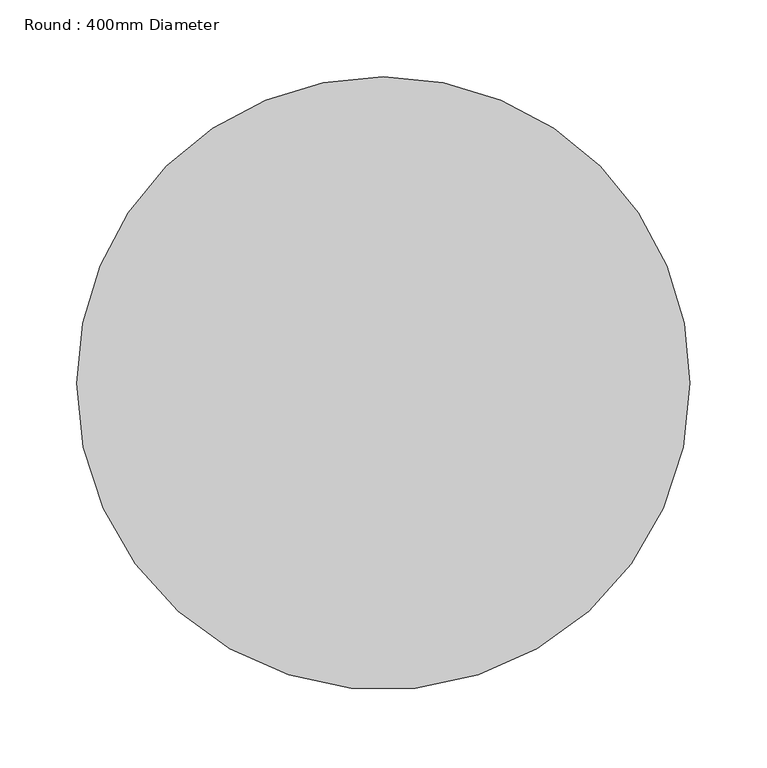
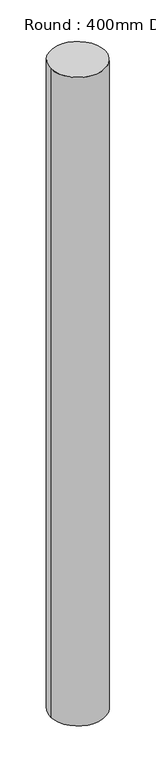
"""IFC4 building model written with IfcOpenShell, lengths in millimetres: column geometry, Round : 400mm Diameter."""

from ifc_helpers import new_model, si_unit, point, frame, origin, origin_2d, place, context, project, spatial, circle_curve, trimmed, segment, composite_curve, outline, extrude, source, transform, mapped, element, save


def round_400mm_diameter_fac56cd9(model_context):
    return source(origin(), model_context, "Body", "SweptSolid", [
        extrude(outline(composite_curve([segment(trimmed(circle_curve(origin_2d(), 200.0), [point((200.0, 0.0))], [point((-200.0, 0.0))], False, "CARTESIAN"), True, "CONTINUOUS"), segment(trimmed(circle_curve(origin_2d(), 200.0), [point((-200.0, 0.0))], [point((0.0, 200.0))], False, "CARTESIAN"), True, "CONTINUOUS"), segment(trimmed(circle_curve(origin_2d(), 200.0), [point((0.0, 200.0))], [point((200.0, 0.0))], False, "CARTESIAN"), True, "CONTINUOUS")], self_intersect=False)), frame((0.0, 0.0, 120050.0), z_axis=(0.0, 0.0, 1.0), x_axis=(1.0, 0.0, 0.0)), (0.0, 0.0, 1.0), 5050.0),
    ])


if __name__ == "__main__":
    model = new_model("IFC4")
    model_context = context("Model", 3, world=origin())
    ifc_project = project(units=[si_unit("LENGTHUNIT", "METRE", prefix="MILLI")], contexts=[model_context])
    site = spatial("IfcSite", under=ifc_project)
    building = spatial("IfcBuilding", under=site)
    placement = place(None, origin())
    round_400mm_diameter_shape = round_400mm_diameter_fac56cd9(model_context)
    element("IfcColumn", 1, ObjectType="Round : 400mm Diameter", at=placement, inside=building, context=model_context, shape_type="MappedRepresentation", body=[
        mapped(round_400mm_diameter_shape, transform((0.0, 0.0, 0.0), x_axis=(1.0, 0.0, 0.0), y_axis=(0.0, 1.0, 0.0), z_axis=(0.0, 0.0, 1.0))),
    ])
    save(model, "model.ifc")

# Revit data of these elements
# Type "Round : 400mm Diameter"
#   Keynote = "G"
#   Diameter = 400.00 mm
#   Offset Base = 0.00 mm
#   Offset Top = 0.00 mm
#   built-in parameter 1002110 = 9474192
#   built-in parameter 1002106 = element 3
#   Material = Concrete - Cast In Situ
# Element 1 (IfcColumn, "Round : 400mm Diameter")
#   Materials on its faces: "Concrete - Cast In Situ"
# Materials
#   "Concrete - Cast In Situ": class "Unassigned", colour RGB 255 255 255, transparency 0, Keynote = "E10/132", Cost = 0
